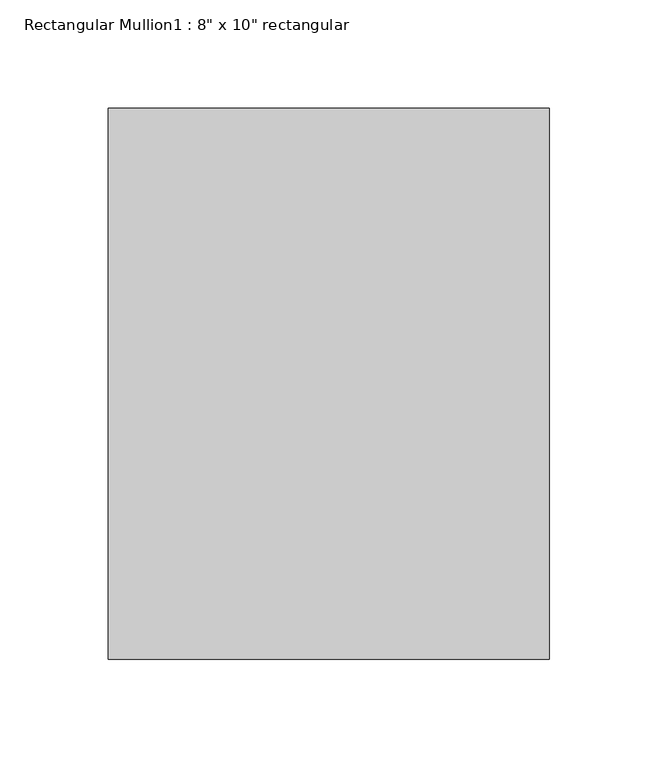
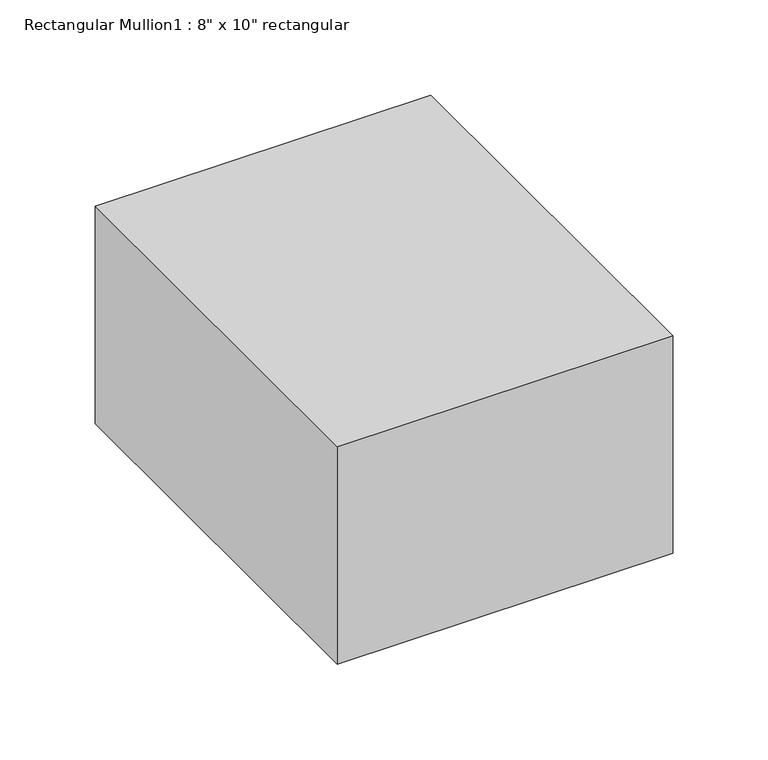
"""IFC4 building model written with IfcOpenShell, lengths in millimetres: member geometry."""

from ifc_helpers import new_model, si_unit, frame, origin, place, context, project, spatial, polyline, outline, extrude, source, transform, mapped, element, save


def member_93925f5f(model_context):
    return source(origin(), model_context, "Body", "SweptSolid", [
        extrude(outline(polyline([(0.0, 127.0), (0.0, -127.0), (-203.2, -127.0), (-203.2, 127.0), (0.0, 127.0)])), frame((0.0, 0.0, -139.2998379), z_axis=(0.0, 0.0, 1.0), x_axis=(1.0, 0.0, 0.0)), (0.0, 0.0, 1.0), 139.2998379),
    ])


if __name__ == "__main__":
    model = new_model("IFC4")
    model_context = context("Model", 3, world=origin())
    ifc_project = project(units=[si_unit("LENGTHUNIT", "METRE", prefix="MILLI")], contexts=[model_context])
    site = spatial("IfcSite", under=ifc_project)
    building = spatial("IfcBuilding", under=site)
    placement = place(None, origin())
    member_shape = member_93925f5f(model_context)
    element("IfcMember", 1, ObjectType="Rectangular Mullion1 : 8\" x 10\" rectangular", at=placement, inside=building, context=model_context, shape_type="MappedRepresentation", body=[
        mapped(member_shape, transform((0.0, 0.0, 0.0), x_axis=(1.0, 0.0, 0.0), y_axis=(0.0, 1.0, 0.0), z_axis=(0.0, 0.0, 1.0))),
    ])
    save(model, "model.ifc")

# Revit data of these elements
# Type "Rectangular Mullion1 : 8\" x 10\" rectangular"
#   built-in parameter 1007304 = 0.833333 (stored number, unit not read)
#   built-in parameter 1007301 = 0.333333 (stored number, unit not read)
#   built-in parameter 1007300 = 0.333333 (stored number, unit not read)
# Element 1 (IfcMember, "Rectangular Mullion1 : 8\" x 10\" rectangular")
#   Materials on its faces: "support-frame"
# Materials
#   "support-frame": class "Unassigned", colour RGB 233 233 233, transparency 0, Cost = 0
